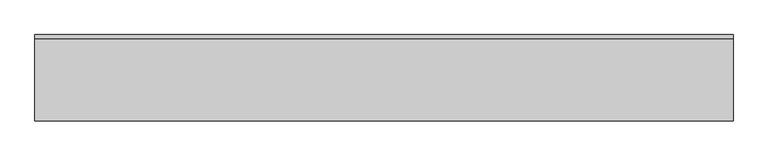
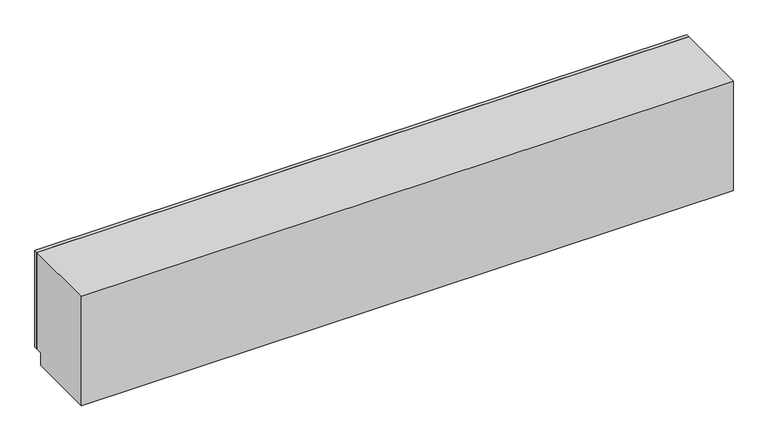
"""IFC4 building model written with IfcOpenShell, lengths in millimetres: furniture geometry, OD_CW_Base Cabinet : OD_CW_Base Cabinet."""

import ifcopenshell
import ifcopenshell.guid

model = None  # the IFC model being written
_history = None  # IfcOwnerHistory: only IFC2X3 demands one
_inside = {}  # id of a spatial element -> (the spatial element, [elements in it])
_under = {}  # id of a project, library or spatial element -> (it, [spatial elements below it])
_declared = {}  # id of a project -> (the project, [libraries it declares])
_typed = {}  # id of a type object -> (the type object, [elements of that type])
_made_of = {}  # id of a material, layer set ... -> (it, [elements and type objects made of it])


def new_model(schema):
    """Start an empty IFC model of exactly this schema.

    Asked for "IFC4X3", IfcOpenShell would pick the latest addendum, in which some entities
    have other attributes; the version numbers below select the first issue.
    IFC2X3 requires an IfcOwnerHistory on every rooted entity: one is made here for all.
    """
    global model, _history
    if schema == "IFC4X3":
        model = ifcopenshell.file(schema_version=(4, 3, 0, 0))
    else:
        model = ifcopenshell.file(schema=schema)
    _inside.clear()
    _under.clear()
    _declared.clear()
    _typed.clear()
    _made_of.clear()
    _history = None
    if model.schema == "IFC2X3":
        org = make("IfcOrganization", Name="unknown")
        user = make(
            "IfcPersonAndOrganization",
            ThePerson=make("IfcPerson", FamilyName="unknown"),
            TheOrganization=org,
        )
        app = make(
            "IfcApplication",
            ApplicationDeveloper=org,
            Version="unknown",
            ApplicationFullName="unknown",
            ApplicationIdentifier="unknown",
        )
        _history = make(
            "IfcOwnerHistory",
            OwningUser=user,
            OwningApplication=app,
            ChangeAction="ADDED",
            CreationDate=0,
        )
    return model


def make(cls, **values):
    """One entity of the class cls with the attributes given. An attribute that is None is left unset."""
    return model.create_entity(
        cls, **{name: value for name, value in values.items() if value is not None}
    )


def rooted(cls, **values):
    """An entity with a GlobalId (a new one), such as an element, a storey or a relation."""
    return make(cls, GlobalId=ifcopenshell.guid.new(), OwnerHistory=_history, **values)


def si_unit(unit_type, name, prefix=None):
    """IfcSIUnit, for example si_unit("LENGTHUNIT", "METRE", prefix="MILLI")."""
    return make("IfcSIUnit", UnitType=unit_type, Prefix=prefix, Name=name)


def assignment(units):
    """IfcUnitAssignment: the units of a project."""
    return None if units is None else make("IfcUnitAssignment", Units=units)


def point(xyz):
    """IfcCartesianPoint."""
    return None if xyz is None else make("IfcCartesianPoint", Coordinates=xyz)


def direction(xyz):
    """IfcDirection."""
    return None if xyz is None else make("IfcDirection", DirectionRatios=xyz)


def frame(location, z_axis=None, x_axis=None):
    """IfcAxis2Placement3D, a coordinate frame: its origin and axes. An axis left out is left unset."""
    return make(
        "IfcAxis2Placement3D",
        Location=point(location),
        Axis=direction(z_axis),
        RefDirection=direction(x_axis),
    )


def origin():
    """The frame at (0, 0, 0) with its axes left unset."""
    return frame((0.0, 0.0, 0.0))


def place(relative_to, where):
    """IfcLocalPlacement: puts the frame where relative to a parent placement (None: the world)."""
    return make(
        "IfcLocalPlacement", PlacementRelTo=relative_to, RelativePlacement=where
    )


def context(
    kind, dimensions, precision=None, world=None, true_north=None, identifier=None
):
    """IfcGeometricRepresentationContext, for example the 3D "Model" context."""
    return make(
        "IfcGeometricRepresentationContext",
        ContextIdentifier=identifier,
        ContextType=kind,
        CoordinateSpaceDimension=dimensions,
        Precision=precision,
        WorldCoordinateSystem=world,
        TrueNorth=true_north,
    )


def project(units=None, contexts=None):
    """IfcProject with its units and contexts."""
    return rooted(
        "IfcProject",
        Name="project",
        RepresentationContexts=contexts,
        UnitsInContext=assignment(units),
    )


def spatial(cls, under=None, at=None, **own):
    """A site, building, storey or space (cls), placed at a placement, below another one or the project."""
    s = rooted(cls, ObjectPlacement=at, **own)
    if under is not None:
        _under.setdefault(under.id(), (under, []))[1].append(s)
    return s


def polyline(points):
    """IfcPolyline through the points."""
    return make("IfcPolyline", Points=[point(p) for p in points])


def outline(outer, holes=None, kind="AREA"):
    """IfcArbitraryClosedProfileDef: a profile drawn as a closed curve; with holes, ...WithVoids."""
    if holes is None:
        return make("IfcArbitraryClosedProfileDef", ProfileType=kind, OuterCurve=outer)
    return make(
        "IfcArbitraryProfileDefWithVoids",
        ProfileType=kind,
        OuterCurve=outer,
        InnerCurves=holes,
    )


def extrude(swept, where, along, depth):
    """IfcExtrudedAreaSolid: the profile swept, set in the frame where, extruded along a direction by depth."""
    return make(
        "IfcExtrudedAreaSolid",
        SweptArea=swept,
        Position=where,
        ExtrudedDirection=direction(along),
        Depth=depth,
    )


def shape(context_of_items, identifier, shape_type, items):
    """IfcShapeRepresentation: the items that make up one representation, for example the "Body"."""
    return make(
        "IfcShapeRepresentation",
        ContextOfItems=context_of_items,
        RepresentationIdentifier=identifier,
        RepresentationType=shape_type,
        Items=items,
    )


def source(mapping_origin, context_of_items, identifier, shape_type, items):
    """IfcRepresentationMap: a shape defined once, which mapped items show again and again."""
    return make(
        "IfcRepresentationMap",
        MappingOrigin=mapping_origin,
        MappedRepresentation=shape(context_of_items, identifier, shape_type, items),
    )


def transform(
    local_origin,
    x_axis=None,
    y_axis=None,
    z_axis=None,
    scale=None,
    scale2=None,
    scale3=None,
    uniform=True,
):
    """IfcCartesianTransformationOperator3D, or its non-uniform kind. x_axis, y_axis, z_axis: its Axis1, 2, 3."""
    if uniform:
        return make(
            "IfcCartesianTransformationOperator3D",
            Axis1=direction(x_axis),
            Axis2=direction(y_axis),
            LocalOrigin=point(local_origin),
            Scale=scale,
            Axis3=direction(z_axis),
        )
    return make(
        "IfcCartesianTransformationOperator3DnonUniform",
        Axis1=direction(x_axis),
        Axis2=direction(y_axis),
        LocalOrigin=point(local_origin),
        Scale=scale,
        Axis3=direction(z_axis),
        Scale2=scale2,
        Scale3=scale3,
    )


def mapped(mapping_source, mapping_target):
    """IfcMappedItem: shows the shape of a source again, moved by a transform."""
    return make(
        "IfcMappedItem", MappingSource=mapping_source, MappingTarget=mapping_target
    )


def made_of(thing, what):
    """Note that an element or type object is made of a material, layer set ...; save() writes the relation."""
    if what is not None:
        _made_of.setdefault(what.id(), (what, []))[1].append(thing)
    return thing


def element(
    cls,
    number,
    at=None,
    inside=None,
    cuts=None,
    type_object=None,
    material=None,
    context=None,
    identifier="Body",
    shape_type=None,
    held_by="IfcProductDefinitionShape",
    body=None,
    shapes=None,
    **own,
):
    """One element of the class cls, such as IfcWall. Its Tag is "e" and its number.

    at: its placement. inside: the storey or other place that contains it. cuts: it is an
    opening in that element (IfcRelVoidsElement). A single representation is given by context,
    identifier, shape_type and body (its items); several are given by shapes. held_by: the class
    of the entity that holds the representations. save() writes the other relations.
    """
    e = rooted(cls, Tag="e%d" % number, ObjectPlacement=at, **own)
    if body is not None:
        shapes = [shape(context, identifier, shape_type, body)]
    if shapes is not None:
        e.Representation = make(held_by, Representations=shapes)
    if inside is not None:
        _inside.setdefault(inside.id(), (inside, []))[1].append(e)
    if cuts is not None:
        rooted(
            "IfcRelVoidsElement", RelatingBuildingElement=cuts, RelatedOpeningElement=e
        )
    if type_object is not None:
        _typed.setdefault(type_object.id(), (type_object, []))[1].append(e)
    return made_of(e, material)


def aggregate(whole, parts):
    """IfcRelAggregates: a whole, such as a stair, and the parts it consists of."""
    return rooted("IfcRelAggregates", RelatingObject=whole, RelatedObjects=parts)


def save(model, path):
    """Write the relations noted so far, then the file.

    IfcRelAggregates (storeys below a building ...), IfcRelContainedInSpatialStructure (elements
    in a storey), IfcRelDefinesByType, IfcRelAssociatesMaterial and IfcRelDeclares: one each for
    every whole, place, type object, material and project.
    """
    for whole, parts in _under.values():
        aggregate(whole, parts)
    for where, things in _inside.values():
        rooted(
            "IfcRelContainedInSpatialStructure",
            RelatedElements=things,
            RelatingStructure=where,
        )
    for kind, things in _typed.values():
        rooted("IfcRelDefinesByType", RelatedObjects=things, RelatingType=kind)
    for what, things in _made_of.values():
        rooted("IfcRelAssociatesMaterial", RelatedObjects=things, RelatingMaterial=what)
    for by, libraries in _declared.values():
        rooted("IfcRelDeclares", RelatingContext=by, RelatedDefinitions=libraries)
    model.write(path)


def furniture_dcd515c4(model_context):
    return source(origin(), model_context, "Body", "SweptSolid", [
        extrude(outline(polyline([(18.7377049, -25.4), (18.7377049, 0.0), (4954.5958279, 0.0), (4954.5958279, -25.4), (18.7377049, -25.4)])), frame((0.0, 0.0, 101.6), z_axis=(0.0, 0.0, 1.0), x_axis=(1.0, 0.0, 0.0)), (0.0, 0.0, 1.0), 774.7),
        extrude(outline(polyline([(-25.4, 876.3), (-25.4, 101.6), (-76.2, 101.6), (-76.2, 0.0), (-609.6, 0.0), (-609.6, 876.3), (-25.4, 876.3)])), frame((18.7377049, 0.0, 0.0), z_axis=(1.0, 0.0, 0.0), x_axis=(0.0, 1.0, 0.0)), (0.0, 0.0, 1.0), 4935.858123),
    ])


if __name__ == "__main__":
    model = new_model("IFC4")
    model_context = context("Model", 3, world=origin())
    ifc_project = project(units=[si_unit("LENGTHUNIT", "METRE", prefix="MILLI")], contexts=[model_context])
    site = spatial("IfcSite", under=ifc_project)
    building = spatial("IfcBuilding", under=site)
    placement = place(None, origin())
    furniture_shape = furniture_dcd515c4(model_context)
    element("IfcFurniture", 1, ObjectType="OD_CW_Base Cabinet : OD_CW_Base Cabinet", at=placement, inside=building, context=model_context, shape_type="MappedRepresentation", body=[
        mapped(furniture_shape, transform((0.0, 0.0, 0.0), x_axis=(1.0, 0.0, 0.0), y_axis=(0.0, 1.0, 0.0), z_axis=(0.0, 0.0, 1.0))),
    ])
    save(model, "model.ifc")

# Revit data of these elements
# Type "OD_CW_Base Cabinet : OD_CW_Base Cabinet"
#   OD_CW_Width [instance default] = 2' - 10"
#   OD_CW_Length [instance default] = 8' - 0"
#   OD_CW_Height [instance default] = 2' - 3"
#   Depth = 2' - 0"
#   Height = 3' - 0"
#   Width = 4' - 0"
#   OD_CW_Material_Front Panel [instance default] = none
#   OD_CW_Material_Body [instance default] = none
# Element 1 (IfcFurniture, "OD_CW_Base Cabinet : OD_CW_Base Cabinet")
#   OD_CW_Width = 2' - 0"
#   OD_CW_Length = 16' - 2.32512"
#   OD_CW_Height = 2' - 10 1/2"
#   Materials on its faces: "CASEWORK"
# Materials
#   "CASEWORK": class "Generic", colour RGB 181 181 181, transparency 0, Cost = 0
